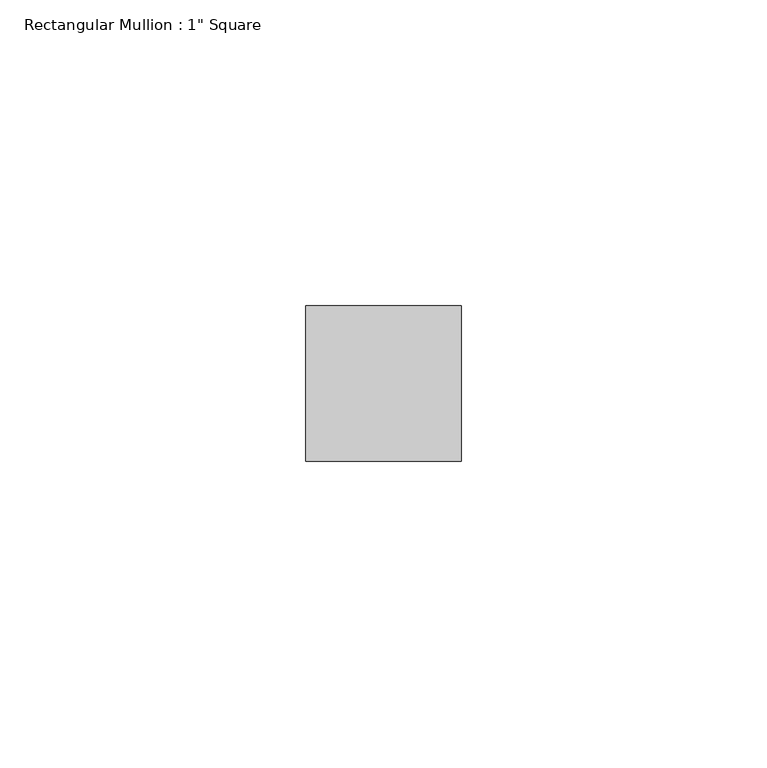
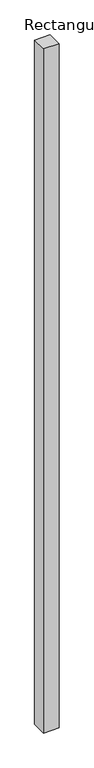
"""IFC4 building model written with IfcOpenShell, lengths in millimetres: member geometry."""

from ifc_helpers import new_model, si_unit, frame, origin, place, context, project, spatial, polyline, outline, extrude, source, transform, mapped, element, save


def member_59ad8a39(model_context):
    return source(origin(), model_context, "Body", "SweptSolid", [
        extrude(outline(polyline([(0.0, 12.7), (0.0, -12.7), (-25.4, -12.7), (-25.4, 12.7), (0.0, 12.7)])), frame((0.0, 0.0, -1193.8), z_axis=(0.0, 0.0, 1.0), x_axis=(1.0, 0.0, 0.0)), (0.0, 0.0, 1.0), 1193.8),
    ])


if __name__ == "__main__":
    model = new_model("IFC4")
    model_context = context("Model", 3, world=origin())
    ifc_project = project(units=[si_unit("LENGTHUNIT", "METRE", prefix="MILLI")], contexts=[model_context])
    site = spatial("IfcSite", under=ifc_project)
    building = spatial("IfcBuilding", under=site)
    placement = place(None, origin())
    member_shape = member_59ad8a39(model_context)
    element("IfcMember", 1, ObjectType="Rectangular Mullion : 1\" Square", at=placement, inside=building, context=model_context, shape_type="MappedRepresentation", body=[
        mapped(member_shape, transform((0.0, 0.0, 0.0), x_axis=(1.0, 0.0, 0.0), y_axis=(0.0, 1.0, 0.0), z_axis=(0.0, 0.0, 1.0))),
    ])
    save(model, "model.ifc")

# Revit data of these elements
# Type "Rectangular Mullion : 1\" Square"
#   built-in parameter 1007304 = 0.0833333 (stored number, unit not read)
#   built-in parameter 1007301 = 0.0416667 (stored number, unit not read)
#   built-in parameter 1007300 = 0.0416667 (stored number, unit not read)
# Element 1 (IfcMember, "Rectangular Mullion : 1\" Square")
#   Materials on its faces: "Metal - Aluminum"
# Materials
#   "Metal - Aluminum": class "Metal", colour RGB 247 247 247, transparency 0
